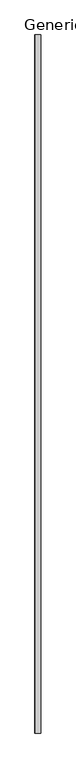
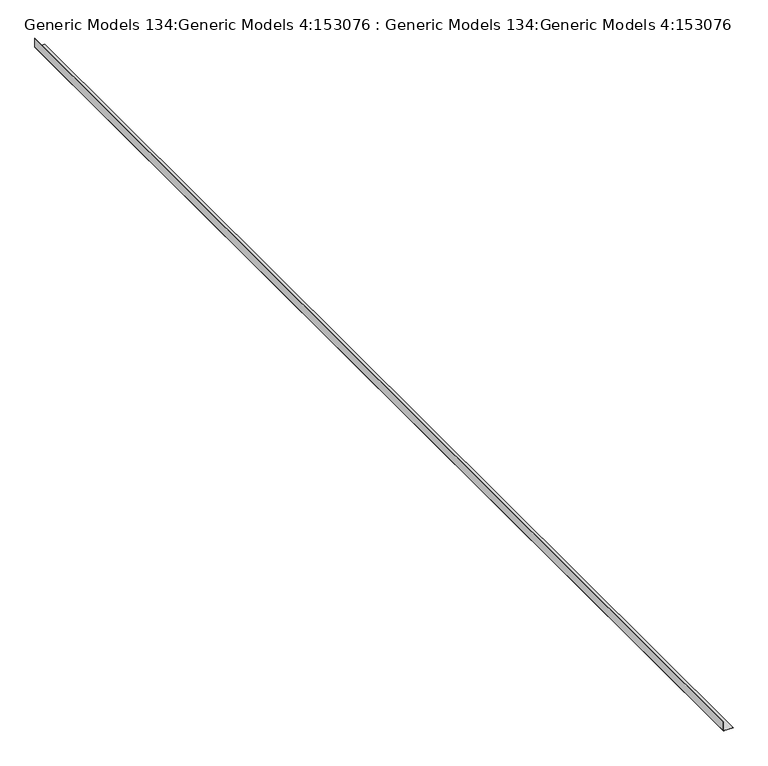
"""IFC4 building model written with IfcOpenShell, lengths in millimetres: proxy geometry, Generic Models 134:Generic Models 4:153076 : Generic Models 134:Generic Models 4:153076."""

from ifc_helpers import new_model, si_unit, frame, origin, place, context, project, spatial, polyline, outline, extrude, source, transform, mapped, element, save


def generic_models_134_generic_models_4_153076_generic_models_71ef999e(model_context):
    return source(origin(), model_context, "Body", "SweptSolid", [
        extrude(outline(polyline([(3605.6524917, 7389.7173492), (3608.826803, 7237.3504114), (3761.226803, 7237.3504114), (3761.226803, 7236.5566614), (3608.0494172, 7236.5566614), (3604.8589139, 7389.7008163), (3605.6524917, 7389.7173492)])), frame((0.0, -6674.7974793, 0.0), z_axis=(0.0, 1.0, 0.0), x_axis=(0.0, 0.0, 1.0)), (0.0, 0.0, 1.0), 18643.6),
    ])


if __name__ == "__main__":
    model = new_model("IFC4")
    model_context = context("Model", 3, world=origin())
    ifc_project = project(units=[si_unit("LENGTHUNIT", "METRE", prefix="MILLI")], contexts=[model_context])
    site = spatial("IfcSite", under=ifc_project)
    building = spatial("IfcBuilding", under=site)
    placement = place(None, origin())
    generic_models_134_generic_models_4_153076_generic_models_shape = generic_models_134_generic_models_4_153076_generic_models_71ef999e(model_context)
    element("IfcBuildingElementProxy", 1, Name="Generic Models 134:Generic Models 4:153076 : Generic Models 134:Generic Models 4:153076", ObjectType="Generic Models 134:Generic Models 4:153076 : Generic Models 134:Generic Models 4:153076", at=placement, inside=building, context=model_context, shape_type="MappedRepresentation", body=[
        mapped(generic_models_134_generic_models_4_153076_generic_models_shape, transform((0.0, 0.0, 0.0), x_axis=(1.0, 0.0, 0.0), y_axis=(0.0, 1.0, 0.0), z_axis=(0.0, 0.0, 1.0))),
    ])
    save(model, "model.ifc")

# Revit data of these elements
# Type "Generic Models 134:Generic Models 4:153076 : Generic Models 134:Generic Models 4:153076"
#   NameOverride = "Generic Models 134:Generic Models 4:153076"
#   ObjectTypeOverride = "Generic Models 134:Generic Models 4"
#   Reference = "Generic Models 4"
#   Category = "Generic Models"
#   Tag = "153076"
# Element 1 (IfcBuildingElementProxy, "Generic Models 134:Generic Models 4:153076 : Generic Models 134:Generic Models 4:153076")
#   Materials on its faces: "_16 GA. COPPER \"L\" FLASHING - (6\" HORZ. LEG - 4\" VERT. LEG) 1711"
# Materials
#   "_16 GA. COPPER \"L\" FLASHING - (6\" HORZ. LEG - 4\" VERT. LEG) 1711": class "Unassigned", colour RGB 156 184 169, transparency 0
